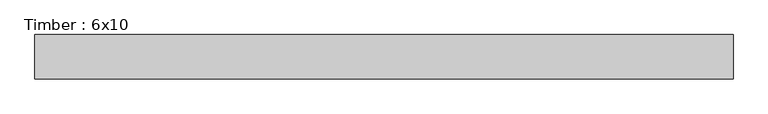
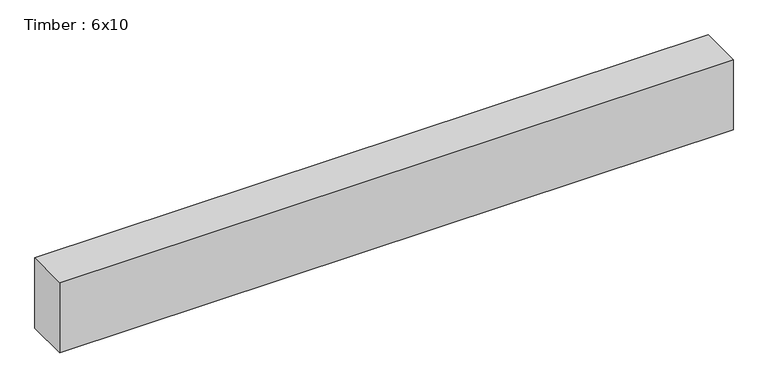
"""IFC4 building model written with IfcOpenShell, lengths in millimetres: beam geometry, Timber : 6x10."""

from ifc_helpers import new_model, si_unit, frame, origin, place, context, project, spatial, polyline, outline, extrude, source, transform, mapped, element, save


def timber_6x10_97aa413e(model_context):
    return source(origin(), model_context, "Body", "SweptSolid", [
        extrude(outline(polyline([(1096.3279, 69.85), (1096.3279, -69.85), (-1091.5816749, -69.85), (-1091.5816749, 69.85), (1096.3279, 69.85)])), frame((0.0, 0.0, -120.65), z_axis=(0.0, 0.0, 1.0), x_axis=(1.0, 0.0, 0.0)), (0.0, 0.0, 1.0), 241.3),
    ])


if __name__ == "__main__":
    model = new_model("IFC4")
    model_context = context("Model", 3, world=origin())
    ifc_project = project(units=[si_unit("LENGTHUNIT", "METRE", prefix="MILLI")], contexts=[model_context])
    site = spatial("IfcSite", under=ifc_project)
    building = spatial("IfcBuilding", under=site)
    placement = place(None, origin())
    timber_6x10_shape = timber_6x10_97aa413e(model_context)
    element("IfcBeam", 1, ObjectType="Timber : 6x10", at=placement, inside=building, context=model_context, shape_type="MappedRepresentation", body=[
        mapped(timber_6x10_shape, transform((0.0, 0.0, 0.0), x_axis=(1.0, 0.0, 0.0), y_axis=(0.0, 1.0, 0.0), z_axis=(0.0, 0.0, 1.0))),
    ])
    save(model, "model.ifc")

# Revit data of these elements
# Type "Timber : 6x10"
#   Assembly Code = "B10"
#   A = 0.362847 SF
#   Length [instance default] = 5' - 0"
#   b = 0' - 5 1/2"
#   d = 0' - 9 1/2"
#   Structural Material [instance default] = Softwood, Lumber
# Element 1 (IfcBeam, "Timber : 6x10")
#   Materials on its faces: "Softwood, Lumber"
# Materials
#   "Softwood, Lumber": class "Wood", colour RGB 144 113 62, transparency 0, Description = "Pinus Echinata", Cost = 0
